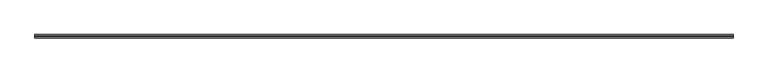
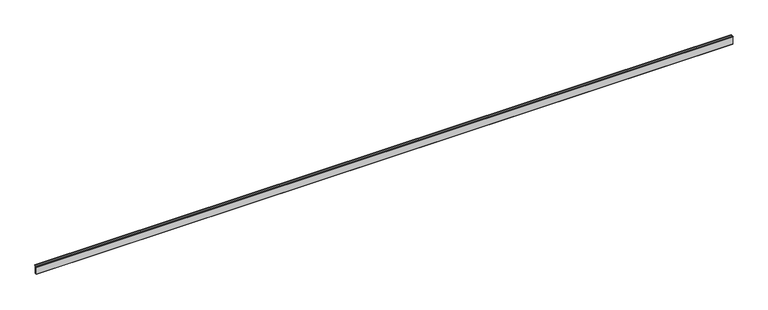
"""IFC4 building model written with IfcOpenShell, lengths in millimetres: railing geometry, ML_Perfil U de embutir : ML_Perfil U de embutir."""

import ifcopenshell
import ifcopenshell.guid

model = None  # the IFC model being written
_history = None  # IfcOwnerHistory: only IFC2X3 demands one
_inside = {}  # id of a spatial element -> (the spatial element, [elements in it])
_under = {}  # id of a project, library or spatial element -> (it, [spatial elements below it])
_declared = {}  # id of a project -> (the project, [libraries it declares])
_typed = {}  # id of a type object -> (the type object, [elements of that type])
_made_of = {}  # id of a material, layer set ... -> (it, [elements and type objects made of it])


def new_model(schema):
    """Start an empty IFC model of exactly this schema.

    Asked for "IFC4X3", IfcOpenShell would pick the latest addendum, in which some entities
    have other attributes; the version numbers below select the first issue.
    IFC2X3 requires an IfcOwnerHistory on every rooted entity: one is made here for all.
    """
    global model, _history
    if schema == "IFC4X3":
        model = ifcopenshell.file(schema_version=(4, 3, 0, 0))
    else:
        model = ifcopenshell.file(schema=schema)
    _inside.clear()
    _under.clear()
    _declared.clear()
    _typed.clear()
    _made_of.clear()
    _history = None
    if model.schema == "IFC2X3":
        org = make("IfcOrganization", Name="unknown")
        user = make(
            "IfcPersonAndOrganization",
            ThePerson=make("IfcPerson", FamilyName="unknown"),
            TheOrganization=org,
        )
        app = make(
            "IfcApplication",
            ApplicationDeveloper=org,
            Version="unknown",
            ApplicationFullName="unknown",
            ApplicationIdentifier="unknown",
        )
        _history = make(
            "IfcOwnerHistory",
            OwningUser=user,
            OwningApplication=app,
            ChangeAction="ADDED",
            CreationDate=0,
        )
    return model


def make(cls, **values):
    """One entity of the class cls with the attributes given. An attribute that is None is left unset."""
    return model.create_entity(
        cls, **{name: value for name, value in values.items() if value is not None}
    )


def rooted(cls, **values):
    """An entity with a GlobalId (a new one), such as an element, a storey or a relation."""
    return make(cls, GlobalId=ifcopenshell.guid.new(), OwnerHistory=_history, **values)


def si_unit(unit_type, name, prefix=None):
    """IfcSIUnit, for example si_unit("LENGTHUNIT", "METRE", prefix="MILLI")."""
    return make("IfcSIUnit", UnitType=unit_type, Prefix=prefix, Name=name)


def assignment(units):
    """IfcUnitAssignment: the units of a project."""
    return None if units is None else make("IfcUnitAssignment", Units=units)


def point(xyz):
    """IfcCartesianPoint."""
    return None if xyz is None else make("IfcCartesianPoint", Coordinates=xyz)


def direction(xyz):
    """IfcDirection."""
    return None if xyz is None else make("IfcDirection", DirectionRatios=xyz)


def frame(location, z_axis=None, x_axis=None):
    """IfcAxis2Placement3D, a coordinate frame: its origin and axes. An axis left out is left unset."""
    return make(
        "IfcAxis2Placement3D",
        Location=point(location),
        Axis=direction(z_axis),
        RefDirection=direction(x_axis),
    )


def origin():
    """The frame at (0, 0, 0) with its axes left unset."""
    return frame((0.0, 0.0, 0.0))


def place(relative_to, where):
    """IfcLocalPlacement: puts the frame where relative to a parent placement (None: the world)."""
    return make(
        "IfcLocalPlacement", PlacementRelTo=relative_to, RelativePlacement=where
    )


def context(
    kind, dimensions, precision=None, world=None, true_north=None, identifier=None
):
    """IfcGeometricRepresentationContext, for example the 3D "Model" context."""
    return make(
        "IfcGeometricRepresentationContext",
        ContextIdentifier=identifier,
        ContextType=kind,
        CoordinateSpaceDimension=dimensions,
        Precision=precision,
        WorldCoordinateSystem=world,
        TrueNorth=true_north,
    )


def project(units=None, contexts=None):
    """IfcProject with its units and contexts."""
    return rooted(
        "IfcProject",
        Name="project",
        RepresentationContexts=contexts,
        UnitsInContext=assignment(units),
    )


def spatial(cls, under=None, at=None, **own):
    """A site, building, storey or space (cls), placed at a placement, below another one or the project."""
    s = rooted(cls, ObjectPlacement=at, **own)
    if under is not None:
        _under.setdefault(under.id(), (under, []))[1].append(s)
    return s


def polyline(points):
    """IfcPolyline through the points."""
    return make("IfcPolyline", Points=[point(p) for p in points])


def outline(outer, holes=None, kind="AREA"):
    """IfcArbitraryClosedProfileDef: a profile drawn as a closed curve; with holes, ...WithVoids."""
    if holes is None:
        return make("IfcArbitraryClosedProfileDef", ProfileType=kind, OuterCurve=outer)
    return make(
        "IfcArbitraryProfileDefWithVoids",
        ProfileType=kind,
        OuterCurve=outer,
        InnerCurves=holes,
    )


def extrude(swept, where, along, depth):
    """IfcExtrudedAreaSolid: the profile swept, set in the frame where, extruded along a direction by depth."""
    return make(
        "IfcExtrudedAreaSolid",
        SweptArea=swept,
        Position=where,
        ExtrudedDirection=direction(along),
        Depth=depth,
    )


def shape(context_of_items, identifier, shape_type, items):
    """IfcShapeRepresentation: the items that make up one representation, for example the "Body"."""
    return make(
        "IfcShapeRepresentation",
        ContextOfItems=context_of_items,
        RepresentationIdentifier=identifier,
        RepresentationType=shape_type,
        Items=items,
    )


def source(mapping_origin, context_of_items, identifier, shape_type, items):
    """IfcRepresentationMap: a shape defined once, which mapped items show again and again."""
    return make(
        "IfcRepresentationMap",
        MappingOrigin=mapping_origin,
        MappedRepresentation=shape(context_of_items, identifier, shape_type, items),
    )


def transform(
    local_origin,
    x_axis=None,
    y_axis=None,
    z_axis=None,
    scale=None,
    scale2=None,
    scale3=None,
    uniform=True,
):
    """IfcCartesianTransformationOperator3D, or its non-uniform kind. x_axis, y_axis, z_axis: its Axis1, 2, 3."""
    if uniform:
        return make(
            "IfcCartesianTransformationOperator3D",
            Axis1=direction(x_axis),
            Axis2=direction(y_axis),
            LocalOrigin=point(local_origin),
            Scale=scale,
            Axis3=direction(z_axis),
        )
    return make(
        "IfcCartesianTransformationOperator3DnonUniform",
        Axis1=direction(x_axis),
        Axis2=direction(y_axis),
        LocalOrigin=point(local_origin),
        Scale=scale,
        Axis3=direction(z_axis),
        Scale2=scale2,
        Scale3=scale3,
    )


def mapped(mapping_source, mapping_target):
    """IfcMappedItem: shows the shape of a source again, moved by a transform."""
    return make(
        "IfcMappedItem", MappingSource=mapping_source, MappingTarget=mapping_target
    )


def made_of(thing, what):
    """Note that an element or type object is made of a material, layer set ...; save() writes the relation."""
    if what is not None:
        _made_of.setdefault(what.id(), (what, []))[1].append(thing)
    return thing


def element(
    cls,
    number,
    at=None,
    inside=None,
    cuts=None,
    type_object=None,
    material=None,
    context=None,
    identifier="Body",
    shape_type=None,
    held_by="IfcProductDefinitionShape",
    body=None,
    shapes=None,
    **own,
):
    """One element of the class cls, such as IfcWall. Its Tag is "e" and its number.

    at: its placement. inside: the storey or other place that contains it. cuts: it is an
    opening in that element (IfcRelVoidsElement). A single representation is given by context,
    identifier, shape_type and body (its items); several are given by shapes. held_by: the class
    of the entity that holds the representations. save() writes the other relations.
    """
    e = rooted(cls, Tag="e%d" % number, ObjectPlacement=at, **own)
    if body is not None:
        shapes = [shape(context, identifier, shape_type, body)]
    if shapes is not None:
        e.Representation = make(held_by, Representations=shapes)
    if inside is not None:
        _inside.setdefault(inside.id(), (inside, []))[1].append(e)
    if cuts is not None:
        rooted(
            "IfcRelVoidsElement", RelatingBuildingElement=cuts, RelatedOpeningElement=e
        )
    if type_object is not None:
        _typed.setdefault(type_object.id(), (type_object, []))[1].append(e)
    return made_of(e, material)


def aggregate(whole, parts):
    """IfcRelAggregates: a whole, such as a stair, and the parts it consists of."""
    return rooted("IfcRelAggregates", RelatingObject=whole, RelatedObjects=parts)


def save(model, path):
    """Write the relations noted so far, then the file.

    IfcRelAggregates (storeys below a building ...), IfcRelContainedInSpatialStructure (elements
    in a storey), IfcRelDefinesByType, IfcRelAssociatesMaterial and IfcRelDeclares: one each for
    every whole, place, type object, material and project.
    """
    for whole, parts in _under.values():
        aggregate(whole, parts)
    for where, things in _inside.values():
        rooted(
            "IfcRelContainedInSpatialStructure",
            RelatedElements=things,
            RelatingStructure=where,
        )
    for kind, things in _typed.values():
        rooted("IfcRelDefinesByType", RelatedObjects=things, RelatingType=kind)
    for what, things in _made_of.values():
        rooted("IfcRelAssociatesMaterial", RelatedObjects=things, RelatingMaterial=what)
    for by, libraries in _declared.values():
        rooted("IfcRelDeclares", RelatingContext=by, RelatedDefinitions=libraries)
    model.write(path)


def railing_3a0e213f(model_context):
    return source(origin(), model_context, "Body", "SweptSolid", [
        extrude(outline(polyline([(1832.4523952, 3702.0), (1832.4523952, 3594.0), (1856.4523952, 3594.0), (1856.4523952, 3702.0), (1866.9523952, 3702.0), (1866.9523952, 3700.0), (1858.4523952, 3700.0), (1858.4523952, 3592.0), (1830.4523952, 3592.0), (1830.4523952, 3700.0), (1821.9523952, 3700.0), (1821.9523952, 3702.0), (1832.4523952, 3702.0)])), frame((-12226.1487231, 0.0, 0.0), z_axis=(1.0, 0.0, 0.0), x_axis=(0.0, 1.0, 0.0)), (0.0, 0.0, 1.0), 9335.0),
    ])


if __name__ == "__main__":
    model = new_model("IFC4")
    model_context = context("Model", 3, world=origin())
    ifc_project = project(units=[si_unit("LENGTHUNIT", "METRE", prefix="MILLI")], contexts=[model_context])
    site = spatial("IfcSite", under=ifc_project)
    building = spatial("IfcBuilding", under=site)
    placement = place(None, origin())
    railing_shape = railing_3a0e213f(model_context)
    element("IfcRailing", 1, ObjectType="ML_Perfil U de embutir : ML_Perfil U de embutir", at=placement, inside=building, context=model_context, shape_type="MappedRepresentation", body=[
        mapped(railing_shape, transform((0.0, 0.0, 0.0), x_axis=(1.0, 0.0, 0.0), y_axis=(0.0, 1.0, 0.0), z_axis=(0.0, 0.0, 1.0))),
    ])
    save(model, "model.ifc")

# Revit data of these elements
# Type "ML_Perfil U de embutir : ML_Perfil U de embutir"
#   ME_Compr [instance default] = 9.335 m
#   ME_Material Perfil [instance default] = .ALUMÍNIO COM PINTURA ELETROSTÁTICA BRANCA
# Element 1 (IfcRailing, "ML_Perfil U de embutir : ML_Perfil U de embutir")
#   Materials on its faces: ".ALUMÍNIO COM PINTURA ELETROSTÁTICA BRANCA"
# Materials
#   ".ALUMÍNIO COM PINTURA ELETROSTÁTICA BRANCA": class "CC_METAIS", colour RGB 241 241 241, transparency 0, Cost = 0
